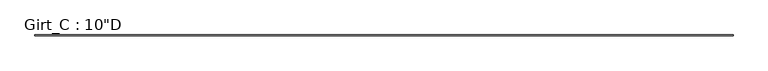
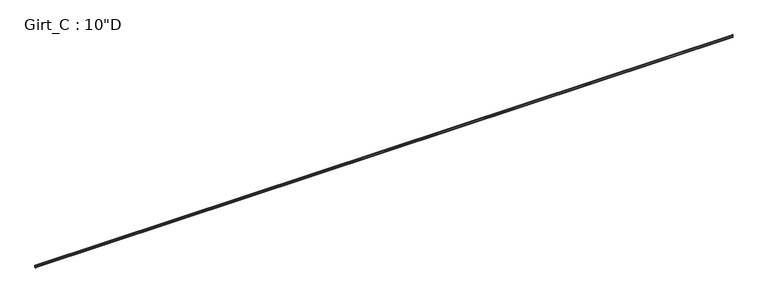
"""IFC4 building model written with IfcOpenShell, lengths in millimetres: beam geometry."""

from ifc_helpers import new_model, si_unit, point, frame, frame_2d, origin, place, context, project, spatial, polyline, circle_curve, trimmed, segment, composite_curve, outline, extrude, source, transform, mapped, element, save


def beam_031b6906(model_context):
    return source(origin(), model_context, "Body", "SweptSolid", [
        extrude(outline(composite_curve([segment(polyline([(-87.5109375, 127.0), (-3.3734375, 127.0)]), True, "CONTINUOUS"), segment(trimmed(circle_curve(frame_2d((-3.3734375, 122.2375)), 4.7625), [point((-3.3734375, 127.0))], [point((1.3890625, 122.2375))], False, "CARTESIAN"), True, "CONTINUOUS"), segment(polyline([(1.3890625, 122.2375), (1.3890625, -122.2375)]), True, "CONTINUOUS"), segment(trimmed(circle_curve(frame_2d((-3.3734375, -122.2375)), 4.7625), [point((1.3890625, -122.2375))], [point((-3.3734375, -127.0))], False, "CARTESIAN"), True, "CONTINUOUS"), segment(polyline([(-3.3734375, -127.0), (-87.5109375, -127.0), (-99.7792647, -112.379177), (-97.6510975, -110.5934327), (-86.2154765, -124.221875), (-3.2694106, -124.221875)]), True, "CONTINUOUS"), segment(trimmed(circle_curve(frame_2d((-3.3748024, -122.2389339)), 1.9857399), [point((-3.2694106, -124.221875))], [point((-1.3890625, -122.2389339))], True, "CARTESIAN"), True, "CONTINUOUS"), segment(polyline([(-1.3890625, -122.2389339), (-1.3890625, 122.2381931)]), True, "CONTINUOUS"), segment(trimmed(circle_curve(frame_2d((-3.3741066, 122.2381931)), 1.9850441), [point((-1.3890625, 122.2381931))], [point((-3.3005807, 124.221875))], True, "CARTESIAN"), True, "CONTINUOUS"), segment(polyline([(-3.3005807, 124.221875), (-86.2154765, 124.221875), (-97.6278742, 110.621109), (-99.7560415, 112.4068534), (-87.5109375, 127.0)]), True, "CONTINUOUS")], self_intersect=False)), frame((-43929.3, 0.0, 0.0), z_axis=(1.0, 0.0, 0.0), x_axis=(0.0, 1.0, 0.0)), (0.0, 0.0, 1.0), 87960.2),
    ])


if __name__ == "__main__":
    model = new_model("IFC4")
    model_context = context("Model", 3, world=origin())
    ifc_project = project(units=[si_unit("LENGTHUNIT", "METRE", prefix="MILLI")], contexts=[model_context])
    site = spatial("IfcSite", under=ifc_project)
    building = spatial("IfcBuilding", under=site)
    placement = place(None, origin())
    beam_shape = beam_031b6906(model_context)
    element("IfcBeam", 1, ObjectType="Girt_C : 10\"D", at=placement, inside=building, context=model_context, shape_type="MappedRepresentation", body=[
        mapped(beam_shape, transform((0.0, 0.0, 0.0), x_axis=(1.0, 0.0, 0.0), y_axis=(0.0, 1.0, 0.0), z_axis=(0.0, 0.0, 1.0))),
    ])
    save(model, "model.ifc")

# Revit data of these elements
# Type "Girt_C : 10\"D"
#   half leg = 0' - 1 3/4"
#   Web_Thickness = 0' - 0 7/64"
#   Length [instance default] = 10' - 0"
#   Leg_1 = 0' - 3 1/2"
#   Height = 0' - 10"
#   Structural Material [instance default] = none
# Element 1 (IfcBeam, "Girt_C : 10\"D")
#   Structural Material = STRUCTURAL STEEL - SEE STRUCT. DWGS
#   Materials on its faces: "STRUCTURAL STEEL - SEE STRUCT. DWGS"
# Materials
#   "STRUCTURAL STEEL - SEE STRUCT. DWGS": class "Metal", colour RGB 137 146 153, transparency 0, Description = "Steel, mill finish", Cost = 0
